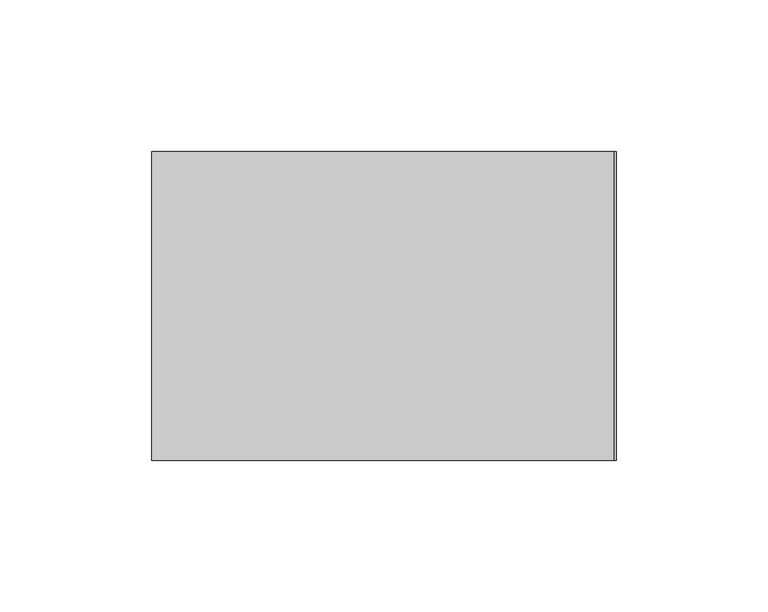
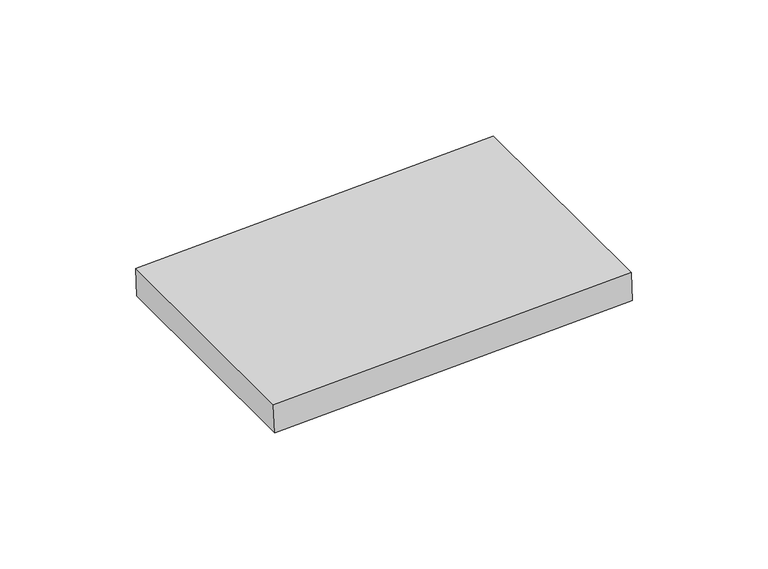
"""IFC4 building model written with IfcOpenShell, lengths in millimetres: proxy geometry, Inner panel:Inner panel:1:Inner panel:1 : Inner panel:Inner panel:300324:2:Inner panel:1:Inner panel:1 : Inner panel:Inner panel:300324:2 : Inner panel:Inner panel:1:Inner panel:1 : Inner panel:Inner panel:300324:300043:47 : Inner panel:Inner panel:1:Inner panel:1 : Inner panel:Inner panel:300324:2:Inner panel:1:Inner panel:1 : Inner panel:Inner panel:300324:2 : Inner panel:Inner panel:1:Inner panel:1 : Inner panel:Inner panel:300324:300043:308120."""

from ifc_helpers import new_model, si_unit, frame, origin, place, context, project, spatial, polyline, outline, extrude, source, transform, mapped, element, save


def generic_models_92468da8(model_context):
    return source(origin(), model_context, "Body", "SweptSolid", [
        extrude(outline(polyline([(0.0, -152.4), (0.0, 0.0), (101.6, 0.0), (101.6, -152.4), (0.0, -152.4)])), frame((560492.7277838, -572644.3413841, 3917.059712), z_axis=(-0.04163054471217779, 0.0, 0.9991330730923521), x_axis=(0.0, 1.0, 0.0)), (0.0, 0.0, 1.0), 12.7),
    ])


if __name__ == "__main__":
    model = new_model("IFC4")
    model_context = context("Model", 3, world=origin())
    ifc_project = project(units=[si_unit("LENGTHUNIT", "METRE", prefix="MILLI")], contexts=[model_context])
    site = spatial("IfcSite", under=ifc_project)
    building = spatial("IfcBuilding", under=site)
    placement = place(None, origin())
    generic_models_shape = generic_models_92468da8(model_context)
    element("IfcBuildingElementProxy", 1, Name="Inner panel:Inner panel:1:Inner panel:1 : Inner panel:Inner panel:300324:2:Inner panel:1:Inner panel:1 : Inner panel:Inner panel:300324:2 : Inner panel:Inner panel:1:Inner panel:1 : Inner panel:Inner panel:300324:300043:47 : Inner panel:Inner panel:1:Inner panel:1 : Inner panel:Inner panel:300324:2:Inner panel:1:Inner panel:1 : Inner panel:Inner panel:300324:2 : Inner panel:Inner panel:1:Inner panel:1 : Inner panel:Inner panel:300324:300043:308120", ObjectType="Inner panel:Inner panel:1:Inner panel:1 : Inner panel:Inner panel:300324:2:Inner panel:1:Inner panel:1 : Inner panel:Inner panel:300324:2 : Inner panel:Inner panel:1:Inner panel:1 : Inner panel:Inner panel:300324:300043:47 : Inner panel:Inner panel:1:Inner panel:1 : Inner panel:Inner panel:300324:2:Inner panel:1:Inner panel:1 : Inner panel:Inner panel:300324:2 : Inner panel:Inner panel:1:Inner panel:1 : Inner panel:Inner panel:300324:300043:308120", at=placement, inside=building, context=model_context, shape_type="MappedRepresentation", body=[
        mapped(generic_models_shape, transform((0.0, 0.0, 0.0), x_axis=(1.0, 0.0, 0.0), y_axis=(0.0, 1.0, 0.0), z_axis=(0.0, 0.0, 1.0))),
    ])
    save(model, "model.ifc")

# Revit data of these elements
# Type "Inner panel:Inner panel:1:Inner panel:1 : Inner panel:Inner panel:300324:2:Inner panel:1:Inner panel:1 : Inner panel:Inner panel:300324:2 : Inner panel:Inner panel:1:Inner panel:1 : Inner panel:Inner panel:300324:300043:47 : Inner panel:Inner panel:1:Inner panel:1 : Inner panel:Inner panel:300324:2:Inner panel:1:Inner panel:1 : Inner panel:Inner panel:300324:2 : Inner panel:Inner panel:1:Inner panel:1 : Inner panel:Inner panel:300324:300043:308120"
#   NameOverride = "Inner panel:Inner panel:1:Inner panel:1 : Inner panel:Inner panel:300324:2:Inner panel:1:Inner panel:1 : Inner panel:Inner panel:300324:2 : Inner panel:Inner panel:1:Inner panel:1 : Inner panel:Inner panel:300324:300043:308120"
#   ObjectTypeOverride = "Inner panel:1:Inner panel:1 : Inner panel:Inner panel:300324:2 : Inner panel:Inner panel:1:Inner panel:1 : Inner panel:Inner panel:300324:300043"
#   Reference = "Inner panel"
#   Tag = "308120"
